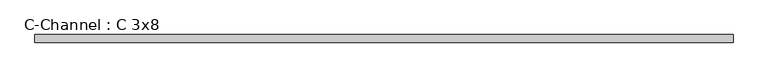
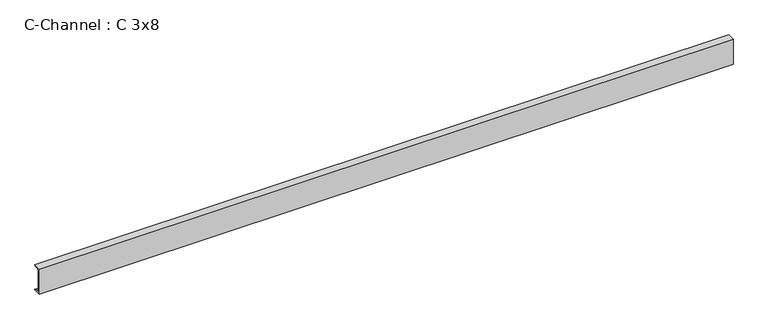
"""IFC4 building model written with IfcOpenShell, lengths in millimetres: beam geometry, C-Channel : C 3x8."""

from ifc_helpers import new_model, si_unit, point, frame, frame_2d, origin, place, context, project, spatial, polyline, circle_curve, trimmed, segment, composite_curve, outline, extrude, source, transform, mapped, element, save


def c_channel_c_3x8_8dc7ccc0(model_context):
    return source(origin(), model_context, "Body", "SweptSolid", [
        extrude(outline(composite_curve([segment(polyline([(-13.5128, 101.6), (44.9072, 101.6)]), True, "CONTINUOUS"), segment(trimmed(circle_curve(frame_2d((35.6108, 101.6)), 9.2964), [point((44.9072, 101.6))], [point((35.6108, 92.3036))], False, "CARTESIAN"), True, "CONTINUOUS"), segment(polyline([(35.6108, 92.3036), (-2.8702, 86.2088084), (-2.8702, -86.2088084), (35.6108, -92.3036)]), True, "CONTINUOUS"), segment(trimmed(circle_curve(frame_2d((35.6108, -101.6)), 9.2964), [point((35.6108, -92.3036))], [point((44.9072, -101.6))], False, "CARTESIAN"), True, "CONTINUOUS"), segment(polyline([(44.9072, -101.6), (-13.5128, -101.6), (-13.5128, 101.6)]), True, "CONTINUOUS")], self_intersect=False)), frame((-2667.0, 0.0, 0.0), z_axis=(1.0, 0.0, 0.0), x_axis=(0.0, 1.0, 0.0)), (0.0, 0.0, 1.0), 5333.9999994),
    ])


if __name__ == "__main__":
    model = new_model("IFC4")
    model_context = context("Model", 3, world=origin())
    ifc_project = project(units=[si_unit("LENGTHUNIT", "METRE", prefix="MILLI")], contexts=[model_context])
    site = spatial("IfcSite", under=ifc_project)
    building = spatial("IfcBuilding", under=site)
    placement = place(None, origin())
    c_channel_c_3x8_shape = c_channel_c_3x8_8dc7ccc0(model_context)
    element("IfcBeam", 1, ObjectType="C-Channel : C 3x8", at=placement, inside=building, context=model_context, shape_type="MappedRepresentation", body=[
        mapped(c_channel_c_3x8_shape, transform((0.0, 0.0, 0.0), x_axis=(1.0, 0.0, 0.0), y_axis=(0.0, 1.0, 0.0), z_axis=(0.0, 0.0, 1.0))),
    ])
    save(model, "model.ifc")

# Revit data of these elements
# Type "C-Channel : C 3x8"
#   Assembly Code = "B10"
#   W = 14.7
#   Length [instance default] = 5' - 0"
#   bf = 0' - 2.3"
#   d = 0' - 8"
#   tf = 0' - 0.366"
#   tw = 0' - 0.419"
#   x = 0' - 0.532"
#   A = 0.0300694 SF
#   Structural Material [instance default] = Steel ASTM A36
# Element 1 (IfcBeam, "C-Channel : C 3x8")
#   Structural Material = Steel ASTM A992
#   Materials on its faces: "Steel ASTM A992"
# Materials
#   "Steel ASTM A36": class "Metal", colour RGB 199 199 199, transparency 0, Description = "Structural steel, ASTM A36 Grade B, mill finish", Cost = 0
#   "Steel ASTM A992": class "Metal", colour RGB 189 187 185, transparency 0, Description = "Structural steel 50ksi", Cost = 0
